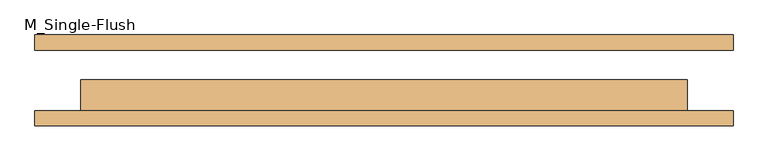
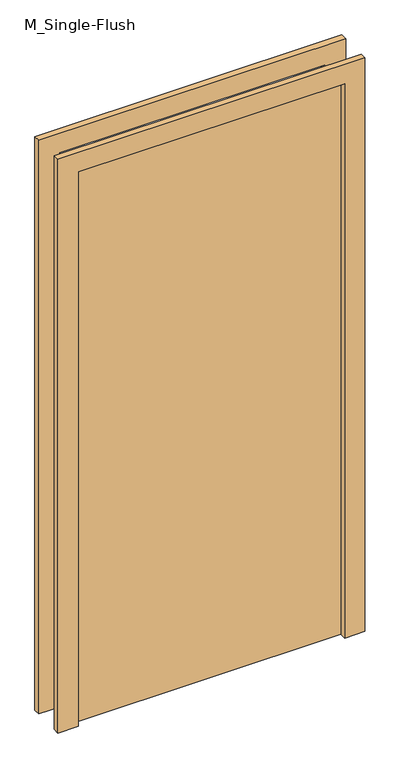
"""IFC4 building model written with IfcOpenShell, lengths in millimetres: door geometry, M_Single-Flush : 100 x 220 Dış Kapı."""

from ifc_helpers import new_model, si_unit, frame, origin, origin_with_axes, place, context, project, spatial, polyline, outline, extrude, source, transform, mapped, element, save


def m_single_flush_349eedbb(model_context):
    return source(origin(), model_context, "Body", "SweptSolid", [
        extrude(outline(polyline([(2276.0, -576.0), (0.0, -576.0), (0.0, -500.0), (2200.0, -500.0), (2200.0, 500.0), (0.0, 500.0), (0.0, 576.0), (2276.0, 576.0), (2276.0, -576.0)])), frame((0.0, -75.0, 0.0), z_axis=(0.0, 1.0, 0.0), x_axis=(0.0, 0.0, 1.0)), (0.0, 0.0, 1.0), 25.0),
        extrude(outline(polyline([(2276.0, 576.0), (2276.0, -576.0), (0.0, -576.0), (0.0, -500.0), (2200.0, -500.0), (2200.0, 500.0), (0.0, 500.0), (0.0, 576.0), (2276.0, 576.0)])), frame((0.0, 50.0, 0.0), z_axis=(0.0, 1.0, 0.0), x_axis=(0.0, 0.0, 1.0)), (0.0, 0.0, 1.0), 25.0),
        extrude(outline(polyline([(500.0, 1.0), (500.0, -50.0), (-500.0, -50.0), (-500.0, 1.0), (500.0, 1.0)])), origin_with_axes(), (0.0, 0.0, 1.0), 2200.0),
    ])


if __name__ == "__main__":
    model = new_model("IFC4")
    model_context = context("Model", 3, world=origin())
    ifc_project = project(units=[si_unit("LENGTHUNIT", "METRE", prefix="MILLI")], contexts=[model_context])
    site = spatial("IfcSite", under=ifc_project)
    building = spatial("IfcBuilding", under=site)
    placement = place(None, origin())
    m_single_flush_shape = m_single_flush_349eedbb(model_context)
    element("IfcDoor", 1, ObjectType="M_Single-Flush : 100 x 220 Dış Kapı", at=placement, inside=building, context=model_context, shape_type="MappedRepresentation", body=[
        mapped(m_single_flush_shape, transform((0.0, 0.0, 0.0), x_axis=(1.0, 0.0, 0.0), y_axis=(0.0, 1.0, 0.0), z_axis=(0.0, 0.0, 1.0))),
    ])
    save(model, "model.ifc")

# Revit data of these elements
# Type "M_Single-Flush : 100 x 220 Dış Kapı"
#   Type Mark = "23"
#   Construction Type Id = "MDOOR"
#   Analytic Construction = "Metal"
#   Thickness = 5.1 cm
#   Thermal Resistance (R) = 0.270117 (m²·K)/W
#   Heat Transfer Coefficient (U) = 3.7021 W/(m²·K)
#   Height = 220 cm
#   Trim Projection Ext = 2.5 cm
#   Trim Projection Int = 2.5 cm
#   Trim Width = 7.6 cm
#   Width = 100 cm
#   Define Thermal Properties by = 1
#   Door Material = Door - Panel
#   Frame Material = Door - Frame
#   Visual Light Transmittance = 0
#   Solar Heat Gain Coefficient = 0
#   Function = (empty or 0)
#   Wall Closure = (empty or 0)
# Element 1 (IfcDoor, "M_Single-Flush : 100 x 220 Dış Kapı")
#   Materials on its faces: "Door - Frame", "Door - Panel"
# Materials
#   "Door - Panel": class "Wood", colour RGB 210 159 95, transparency 0, Cost = 0
#   "Door - Frame": class "Miscellaneous", colour RGB 118 70 51, transparency 0, Cost = 0
